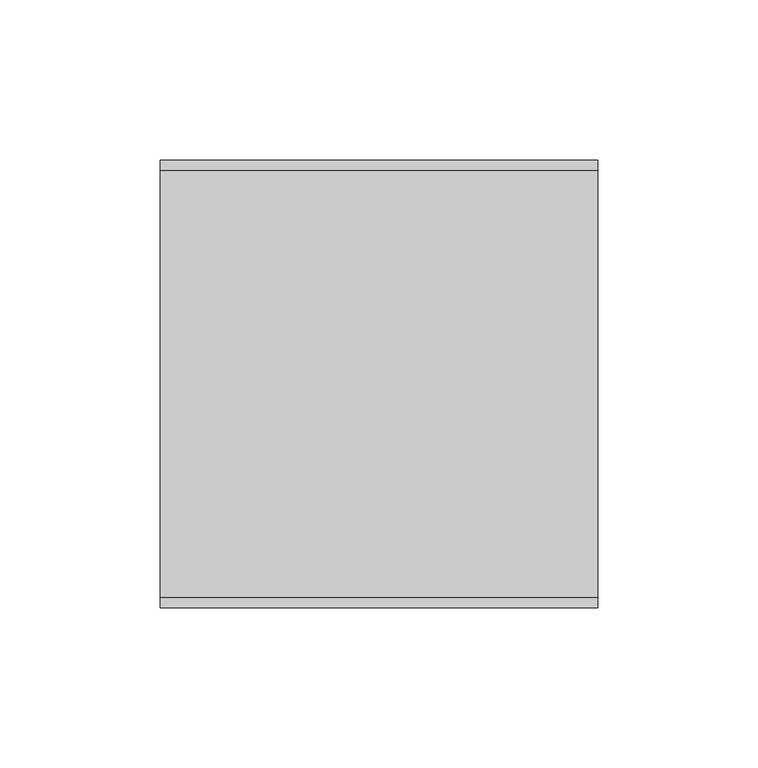
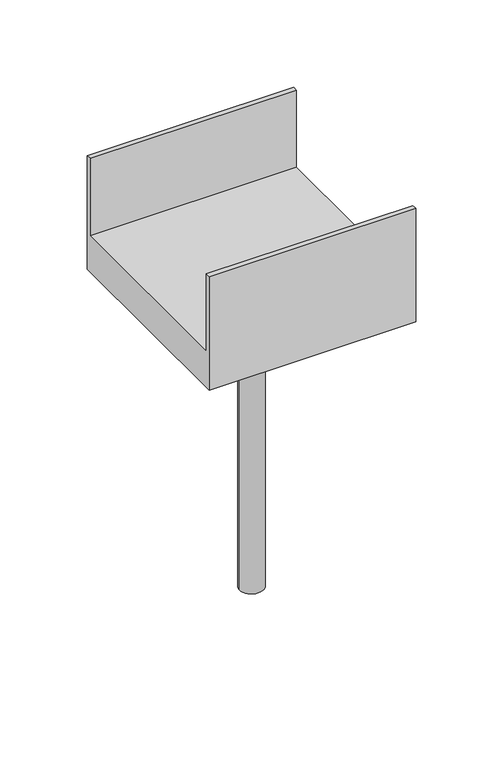
"""IFC4 building model written with IfcOpenShell, lengths in millimetres: fastener geometry."""

from ifc_helpers import new_model, si_unit, point, frame, origin, origin_with_axes, origin_2d, place, context, project, spatial, polyline, circle_curve, trimmed, segment, composite_curve, outline, extrude, source, transform, mapped, element, save


def fastener_d5b4f6b8(model_context):
    return source(origin(), model_context, "Body", "SweptSolid", [
        extrude(outline(composite_curve([segment(trimmed(circle_curve(origin_2d(), 7.9375), [point((-7.9375, 0.0))], [point((7.9375, 0.0))], False, "CARTESIAN"), True, "CONTINUOUS"), segment(trimmed(circle_curve(origin_2d(), 7.9375), [point((7.9375, 0.0))], [point((-7.9375, 0.0))], False, "CARTESIAN"), True, "CONTINUOUS")], self_intersect=False)), frame((0.0, 0.0, -203.2), z_axis=(0.0, 0.0, 1.0), x_axis=(1.0, 0.0, 0.0)), (0.0, 0.0, 1.0), 203.2),
        extrude(outline(polyline([(-11.90625, 6.8740766), (0.0, 13.7481533), (11.90625, 6.8740766), (11.90625, -6.8740766), (0.0, -13.7481533), (-11.90625, -6.8740766), (-11.90625, 6.8740766)])), origin_with_axes(), (0.0, 0.0, 1.0), 11.2117187),
        extrude(outline(polyline([(-69.85, 79.375), (-66.675, 79.375), (-66.675, 25.4), (66.675, 25.4), (66.675, 79.375), (69.85, 79.375), (69.85, 0.0), (-69.85, 0.0), (-69.85, 79.375)])), frame((-68.2625, 0.0, 0.0), z_axis=(1.0, 0.0, 0.0), x_axis=(0.0, 1.0, 0.0)), (0.0, 0.0, 1.0), 136.525),
    ])


if __name__ == "__main__":
    model = new_model("IFC4")
    model_context = context("Model", 3, world=origin())
    ifc_project = project(units=[si_unit("LENGTHUNIT", "METRE", prefix="MILLI")], contexts=[model_context])
    site = spatial("IfcSite", under=ifc_project)
    building = spatial("IfcBuilding", under=site)
    placement = place(None, origin())
    fastener_shape = fastener_d5b4f6b8(model_context)
    element("IfcFastener", 1, ObjectType="SIMPSON - ABA- POST BASE : SIMPSON - ABA66Z W/ 5/8\"X8\" ANCHOR BOLT W/ NON-SHRINK GROUT AT BASE", at=placement, inside=building, context=model_context, shape_type="MappedRepresentation", body=[
        mapped(fastener_shape, transform((0.0, 0.0, 0.0), x_axis=(1.0, 0.0, 0.0), y_axis=(0.0, 1.0, 0.0), z_axis=(0.0, 0.0, 1.0))),
    ])
    save(model, "model.ifc")

# Revit data of these elements
# Type "SIMPSON - ABA- POST BASE : SIMPSON - ABA66Z W/ 5/8\"X8\" ANCHOR BOLT W/ NON-SHRINK GROUT AT BASE"
#   L = 0' - 3"
#   Hole Radius = 0' - 0 3/8"
#   D4 = 0' - 5"
#   D2 = 0' - 5"
#   D1 = 0' - 1 1/2"
#   D3 = 0' - 2 3/4"
#   Ga. = 0' - 0 61/256"
#   W1 & W2 = 0' - 4 1/4"
#   Default Elevation = 4' - 0"
#   Bolt Visibility - 3B = no
#   Bolt Visibility - 3A = no
#   Bolt Visibility - 2B = no
#   Bolt Visibility - 2A = no
#   Bolt Visibility - 1B = no
#   Bolt Visibility - 1A = yes
#   Bolt Visibility = yes
#   Material = ABA66Z W/ 5/8"X8" ANCHOR BOLT W/ NON-SHRINK GROUT AT BASE
#   Bolt Size = element 1605874
#   URL = ""
# Element 1 (IfcFastener, "SIMPSON - ABA- POST BASE : SIMPSON - ABA66Z W/ 5/8\"X8\" ANCHOR BOLT W/ NON-SHRINK GROUT AT BASE")
#   Materials on its faces: "1\" GALV. LAG BOLT (LENGTH = 1/2\" SHY OF GLULAM DEPTH) -  (GALV. THRU BOLT IF PLATE ON OPP. SIDE OF STRUCT MEMBER)", "ABA66Z W/ 5/8\"X8\" ANCHOR BOLT W/ NON-SHRINK GROUT AT BASE"
# Materials
#   "ABA66Z W/ 5/8\"X8\" ANCHOR BOLT W/ NON-SHRINK GROUT AT BASE": class "Generic", colour RGB 232 232 232, transparency 0, Cost = 0
#   "1\" GALV. LAG BOLT (LENGTH = 1/2\" SHY OF GLULAM DEPTH) -  (GALV. THRU BOLT IF PLATE ON OPP. SIDE OF STRUCT MEMBER)": class "Generic", colour RGB 120 120 120, transparency 0, Cost = 0
